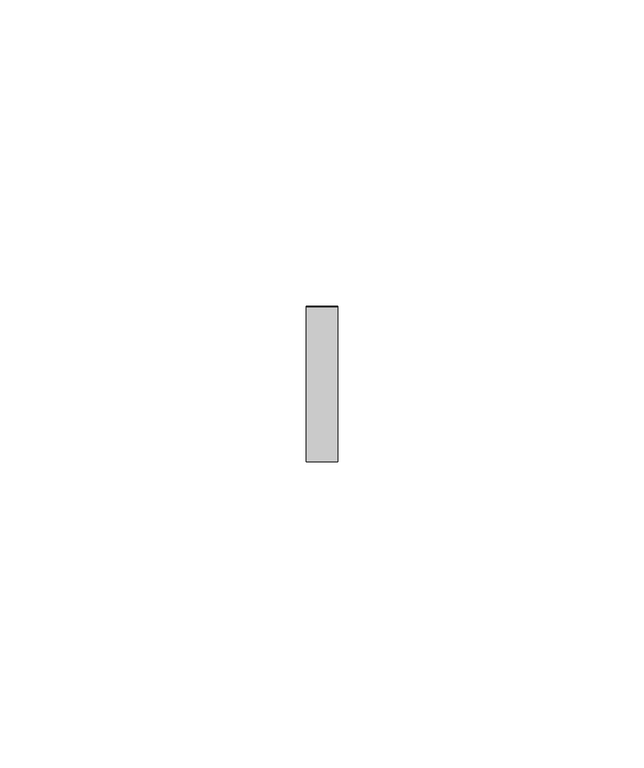
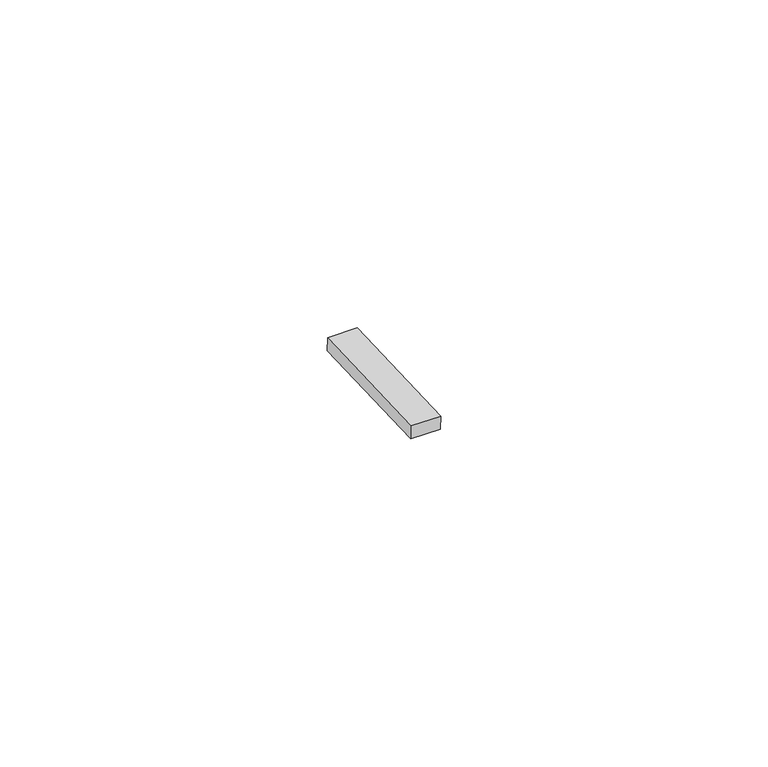
"""IFC4 building model written with IfcOpenShell, lengths in millimetres: proxy geometry, Inner panel:Inner panel:1:Inner panel:1 : Inner panel:Inner panel:300324:2:Inner panel:1:Inner panel:1 : Inner panel:Inner panel:300324:2 : Inner panel:Inner panel:1:Inner panel:1 : Inner panel:Inner panel:300324:300043:142 : Inner panel:Inner panel:1:Inner panel:1 : Inner panel:Inner panel:300324:2:Inner panel:1:Inner panel:1 : Inner panel:Inner panel:300324:2 : Inner panel:Inner panel:1:Inner panel:1 : Inner panel:Inner panel:300324:300043:308120."""

from ifc_helpers import new_model, si_unit, frame, origin, place, context, project, spatial, polyline, outline, extrude, source, transform, mapped, element, save


def generic_models_fc56fcc7(model_context):
    return source(origin(), model_context, "Body", "SweptSolid", [
        extrude(outline(polyline([(0.0, -25.4), (0.0, 0.0), (5.2138089, 0.0), (5.2138089, -25.4), (0.0, -25.4)])), frame((592310.995117, -579790.2297895, 3917.0009179), z_axis=(0.0, -0.041630544712223896, 0.9991330730923502), x_axis=(-1.0, 0.0, 0.0)), (0.0, 0.0, 1.0), 2.4763745),
    ])


if __name__ == "__main__":
    model = new_model("IFC4")
    model_context = context("Model", 3, world=origin())
    ifc_project = project(units=[si_unit("LENGTHUNIT", "METRE", prefix="MILLI")], contexts=[model_context])
    site = spatial("IfcSite", under=ifc_project)
    building = spatial("IfcBuilding", under=site)
    placement = place(None, origin())
    generic_models_shape = generic_models_fc56fcc7(model_context)
    element("IfcBuildingElementProxy", 1, Name="Inner panel:Inner panel:1:Inner panel:1 : Inner panel:Inner panel:300324:2:Inner panel:1:Inner panel:1 : Inner panel:Inner panel:300324:2 : Inner panel:Inner panel:1:Inner panel:1 : Inner panel:Inner panel:300324:300043:142 : Inner panel:Inner panel:1:Inner panel:1 : Inner panel:Inner panel:300324:2:Inner panel:1:Inner panel:1 : Inner panel:Inner panel:300324:2 : Inner panel:Inner panel:1:Inner panel:1 : Inner panel:Inner panel:300324:300043:308120", ObjectType="Inner panel:Inner panel:1:Inner panel:1 : Inner panel:Inner panel:300324:2:Inner panel:1:Inner panel:1 : Inner panel:Inner panel:300324:2 : Inner panel:Inner panel:1:Inner panel:1 : Inner panel:Inner panel:300324:300043:142 : Inner panel:Inner panel:1:Inner panel:1 : Inner panel:Inner panel:300324:2:Inner panel:1:Inner panel:1 : Inner panel:Inner panel:300324:2 : Inner panel:Inner panel:1:Inner panel:1 : Inner panel:Inner panel:300324:300043:308120", at=placement, inside=building, context=model_context, shape_type="MappedRepresentation", body=[
        mapped(generic_models_shape, transform((0.0, 0.0, 0.0), x_axis=(1.0, 0.0, 0.0), y_axis=(0.0, 1.0, 0.0), z_axis=(0.0, 0.0, 1.0))),
    ])
    save(model, "model.ifc")

# Revit data of these elements
# Type "Inner panel:Inner panel:1:Inner panel:1 : Inner panel:Inner panel:300324:2:Inner panel:1:Inner panel:1 : Inner panel:Inner panel:300324:2 : Inner panel:Inner panel:1:Inner panel:1 : Inner panel:Inner panel:300324:300043:142 : Inner panel:Inner panel:1:Inner panel:1 : Inner panel:Inner panel:300324:2:Inner panel:1:Inner panel:1 : Inner panel:Inner panel:300324:2 : Inner panel:Inner panel:1:Inner panel:1 : Inner panel:Inner panel:300324:300043:308120"
#   NameOverride = "Inner panel:Inner panel:1:Inner panel:1 : Inner panel:Inner panel:300324:2:Inner panel:1:Inner panel:1 : Inner panel:Inner panel:300324:2 : Inner panel:Inner panel:1:Inner panel:1 : Inner panel:Inner panel:300324:300043:308120"
#   ObjectTypeOverride = "Inner panel:1:Inner panel:1 : Inner panel:Inner panel:300324:2 : Inner panel:Inner panel:1:Inner panel:1 : Inner panel:Inner panel:300324:300043"
#   Reference = "Inner panel"
#   Tag = "308120"
# Element 1 (IfcBuildingElementProxy, "Inner panel:Inner panel:1:Inner panel:1 : Inner panel:Inner panel:300324:2:Inner panel:1:Inner panel:1 : Inner panel:Inner panel:300324:2 : Inner panel:Inner panel:1:Inner panel:1 : Inner panel:Inner panel:300324:300043:142 : Inner panel:Inner panel:1:Inner panel:1 : Inner panel:Inner panel:300324:2:Inner panel:1:Inner panel:1 : Inner panel:Inner panel:300324:2 : Inner panel:Inner panel:1:Inner panel:1 : Inner panel:Inner panel:300324:300043:308120")
#   Materials on its faces: "AT CLIP - 1\" WIDE NON ABSORBENT, WEATHER-RESISTANT NEOPRENE/EPDM/SBR FOAM"
# Materials
#   "AT CLIP - 1\" WIDE NON ABSORBENT, WEATHER-RESISTANT NEOPRENE/EPDM/SBR FOAM": class "Generic", colour RGB 85 85 85, transparency 0, Cost = 0
